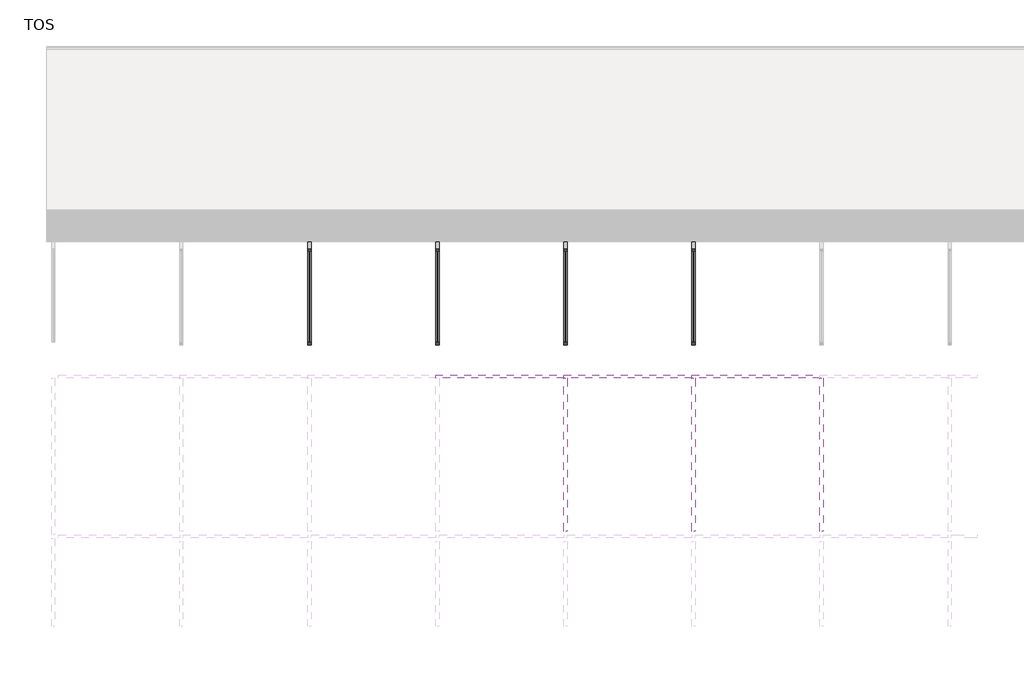
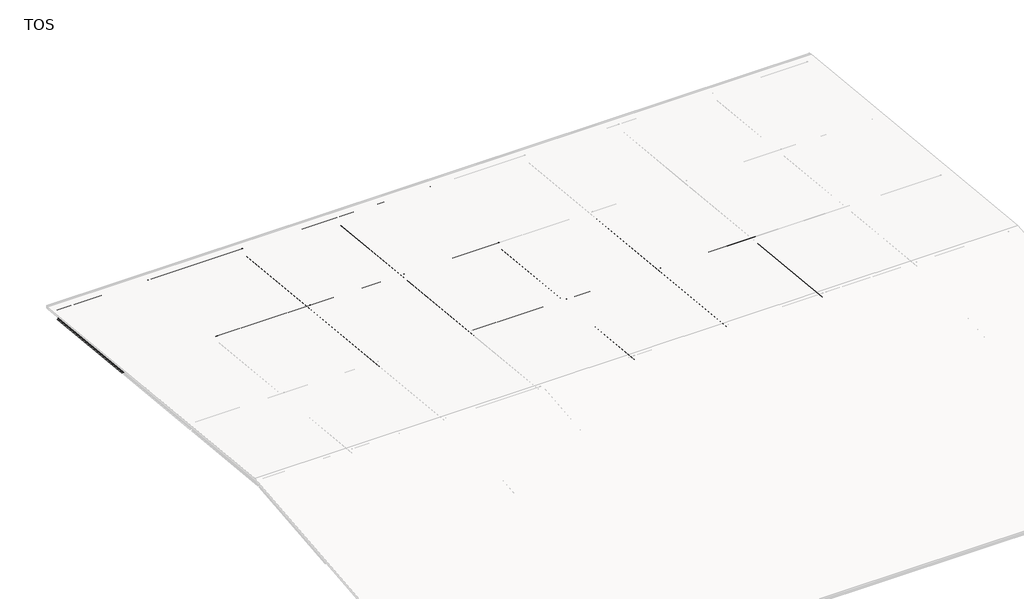
# One storey, part 4 of 5: 22 beams.
"""IFC4 building model written with IfcOpenShell, lengths in millimetres."""

from ifc_helpers import new_model, si_unit, point, frame, frame_2d, origin, place, context, project, spatial, polyline, circle_curve, trimmed, segment, composite_curve, outline, extrude, element, save

model = new_model("IFC4")

# Units and contexts
model_context = context("Model", 3, world=origin())
ifc_project = project(units=[si_unit("LENGTHUNIT", "METRE", prefix="MILLI")], contexts=[model_context])

# Site, building, storey
site = spatial("IfcSite", under=ifc_project)
building = spatial("IfcBuilding", under=site)
storey = spatial("IfcBuildingStorey", under=building, Name="TOS", Elevation=9299.9618634)

# Beams
placement = place(None, origin())
element("IfcBeam", 1, ObjectType="0912_Steel Framing_H-KSD3502 : H_SB_ASB_H-600x200x11x17", at=placement, inside=storey, context=model_context, shape_type="SweptSolid", body=[
    extrude(outline(composite_curve([segment(polyline([(40599.5208589, 10716.9618634), (40599.5208589, 10699.9618634), (40399.5208589, 10699.9618634), (40399.5208589, 10716.9618634), (40472.0208589, 10716.9618634)]), True, "CONTINUOUS"), segment(trimmed(circle_curve(frame_2d((40472.0208589, 10738.9618634)), 22.0), [point((40472.0208589, 10716.9618634))], [point((40494.0208589, 10738.9618634))], True, "CARTESIAN"), True, "CONTINUOUS"), segment(polyline([(40494.0208589, 10738.9618634), (40494.0208589, 11260.9618634)]), True, "CONTINUOUS"), segment(trimmed(circle_curve(frame_2d((40472.0208589, 11260.9618634)), 22.0), [point((40494.0208589, 11260.9618634))], [point((40472.0208589, 11282.9618634))], True, "CARTESIAN"), True, "CONTINUOUS"), segment(polyline([(40472.0208589, 11282.9618634), (40399.5208589, 11282.9618634), (40399.5208589, 11299.9618634), (40599.5208589, 11299.9618634), (40599.5208589, 11282.9618634), (40527.0208589, 11282.9618634)]), True, "CONTINUOUS"), segment(trimmed(circle_curve(frame_2d((40527.0208589, 11260.9618634)), 22.0), [point((40527.0208589, 11282.9618634))], [point((40505.0208589, 11260.9618634))], True, "CARTESIAN"), True, "CONTINUOUS"), segment(polyline([(40505.0208589, 11260.9618634), (40505.0208589, 10738.9618634)]), True, "CONTINUOUS"), segment(trimmed(circle_curve(frame_2d((40527.0208589, 10738.9618634)), 22.0), [point((40505.0208589, 10738.9618634))], [point((40527.0208589, 10716.9618634))], True, "CARTESIAN"), True, "CONTINUOUS"), segment(polyline([(40527.0208589, 10716.9618634), (40599.5208589, 10716.9618634)]), True, "CONTINUOUS")], self_intersect=False)), frame((23900.0, 0.0, 0.0), z_axis=(1.0, 0.0, 0.0), x_axis=(0.0, 1.0, 0.0)), (0.0, 0.0, 1.0), 7987.3),
])
element("IfcBeam", 2, ObjectType="0912_Steel Framing_H-KSD3502 : H_SB_ASB_H-600x200x11x17", at=placement, inside=storey, context=model_context, shape_type="SweptSolid", body=[
    extrude(outline(composite_curve([segment(polyline([(40599.5208589, 10716.9618634), (40599.5208589, 10699.9618634), (40399.5208589, 10699.9618634), (40399.5208589, 10716.9618634), (40472.0208589, 10716.9618634)]), True, "CONTINUOUS"), segment(trimmed(circle_curve(frame_2d((40472.0208589, 10738.9618634)), 22.0), [point((40472.0208589, 10716.9618634))], [point((40494.0208589, 10738.9618634))], True, "CARTESIAN"), True, "CONTINUOUS"), segment(polyline([(40494.0208589, 10738.9618634), (40494.0208589, 11260.9618634)]), True, "CONTINUOUS"), segment(trimmed(circle_curve(frame_2d((40472.0208589, 11260.9618634)), 22.0), [point((40494.0208589, 11260.9618634))], [point((40472.0208589, 11282.9618634))], True, "CARTESIAN"), True, "CONTINUOUS"), segment(polyline([(40472.0208589, 11282.9618634), (40399.5208589, 11282.9618634), (40399.5208589, 11299.9618634), (40599.5208589, 11299.9618634), (40599.5208589, 11282.9618634), (40527.0208589, 11282.9618634)]), True, "CONTINUOUS"), segment(trimmed(circle_curve(frame_2d((40527.0208589, 11260.9618634)), 22.0), [point((40527.0208589, 11282.9618634))], [point((40505.0208589, 11260.9618634))], True, "CARTESIAN"), True, "CONTINUOUS"), segment(polyline([(40505.0208589, 11260.9618634), (40505.0208589, 10738.9618634)]), True, "CONTINUOUS"), segment(trimmed(circle_curve(frame_2d((40527.0208589, 10738.9618634)), 22.0), [point((40505.0208589, 10738.9618634))], [point((40527.0208589, 10716.9618634))], True, "CARTESIAN"), True, "CONTINUOUS"), segment(polyline([(40527.0208589, 10716.9618634), (40599.5208589, 10716.9618634)]), True, "CONTINUOUS")], self_intersect=False)), frame((31900.0, 0.0, 0.0), z_axis=(1.0, 0.0, 0.0), x_axis=(0.0, 1.0, 0.0)), (0.0, 0.0, 1.0), 7987.3),
])
element("IfcBeam", 3, ObjectType="0912_Steel Framing_H-KSD3502 : H_SB_ASB_H-600x200x11x17", at=placement, inside=storey, context=model_context, shape_type="SweptSolid", body=[
    extrude(outline(composite_curve([segment(polyline([(40599.5208589, 10716.9618634), (40599.5208589, 10699.9618634), (40399.5208589, 10699.9618634), (40399.5208589, 10716.9618634), (40472.0208589, 10716.9618634)]), True, "CONTINUOUS"), segment(trimmed(circle_curve(frame_2d((40472.0208589, 10738.9618634)), 22.0), [point((40472.0208589, 10716.9618634))], [point((40494.0208589, 10738.9618634))], True, "CARTESIAN"), True, "CONTINUOUS"), segment(polyline([(40494.0208589, 10738.9618634), (40494.0208589, 11260.9618634)]), True, "CONTINUOUS"), segment(trimmed(circle_curve(frame_2d((40472.0208589, 11260.9618634)), 22.0), [point((40494.0208589, 11260.9618634))], [point((40472.0208589, 11282.9618634))], True, "CARTESIAN"), True, "CONTINUOUS"), segment(polyline([(40472.0208589, 11282.9618634), (40399.5208589, 11282.9618634), (40399.5208589, 11299.9618634), (40599.5208589, 11299.9618634), (40599.5208589, 11282.9618634), (40527.0208589, 11282.9618634)]), True, "CONTINUOUS"), segment(trimmed(circle_curve(frame_2d((40527.0208589, 11260.9618634)), 22.0), [point((40527.0208589, 11282.9618634))], [point((40505.0208589, 11260.9618634))], True, "CARTESIAN"), True, "CONTINUOUS"), segment(polyline([(40505.0208589, 11260.9618634), (40505.0208589, 10738.9618634)]), True, "CONTINUOUS"), segment(trimmed(circle_curve(frame_2d((40527.0208589, 10738.9618634)), 22.0), [point((40505.0208589, 10738.9618634))], [point((40527.0208589, 10716.9618634))], True, "CARTESIAN"), True, "CONTINUOUS"), segment(polyline([(40527.0208589, 10716.9618634), (40599.5208589, 10716.9618634)]), True, "CONTINUOUS")], self_intersect=False)), frame((39900.0, 0.0, 0.0), z_axis=(1.0, 0.0, 0.0), x_axis=(0.0, 1.0, 0.0)), (0.0, 0.0, 1.0), 7987.3),
])
element("IfcBeam", 4, ObjectType="0912_Steel Framing_H-KSD3502 : H_SB_ASB_H-600x200x11x17", at=placement, inside=storey, context=model_context, shape_type="SweptSolid", body=[
    extrude(outline(composite_curve([segment(polyline([(50599.5208589, 9716.9618634), (50599.5208589, 9699.9618634), (50399.5208589, 9699.9618634), (50399.5208589, 9716.9618634), (50472.0208589, 9716.9618634)]), True, "CONTINUOUS"), segment(trimmed(circle_curve(frame_2d((50472.0208589, 9738.9618634)), 22.0), [point((50472.0208589, 9716.9618634))], [point((50494.0208589, 9738.9618634))], True, "CARTESIAN"), True, "CONTINUOUS"), segment(polyline([(50494.0208589, 9738.9618634), (50494.0208589, 10260.9618634)]), True, "CONTINUOUS"), segment(trimmed(circle_curve(frame_2d((50472.0208589, 10260.9618634)), 22.0), [point((50494.0208589, 10260.9618634))], [point((50472.0208589, 10282.9618634))], True, "CARTESIAN"), True, "CONTINUOUS"), segment(polyline([(50472.0208589, 10282.9618634), (50399.5208589, 10282.9618634), (50399.5208589, 10299.9618634), (50599.5208589, 10299.9618634), (50599.5208589, 10282.9618634), (50527.0208589, 10282.9618634)]), True, "CONTINUOUS"), segment(trimmed(circle_curve(frame_2d((50527.0208589, 10260.9618634)), 22.0), [point((50527.0208589, 10282.9618634))], [point((50505.0208589, 10260.9618634))], True, "CARTESIAN"), True, "CONTINUOUS"), segment(polyline([(50505.0208589, 10260.9618634), (50505.0208589, 9738.9618634)]), True, "CONTINUOUS"), segment(trimmed(circle_curve(frame_2d((50527.0208589, 9738.9618634)), 22.0), [point((50505.0208589, 9738.9618634))], [point((50527.0208589, 9716.9618634))], True, "CARTESIAN"), True, "CONTINUOUS"), segment(polyline([(50527.0208589, 9716.9618634), (50599.5208589, 9716.9618634)]), True, "CONTINUOUS")], self_intersect=False)), frame((318.7, 0.0, 0.0), z_axis=(1.0, 0.0, 0.0), x_axis=(0.0, 1.0, 0.0)), (0.0, 0.0, 1.0), 7568.6),
])
element("IfcBeam", 5, ObjectType="0912_Steel Framing_H-KSD3502 : H_SB_ASB_H-600x200x11x17", at=placement, inside=storey, context=model_context, shape_type="SweptSolid", body=[
    extrude(outline(composite_curve([segment(polyline([(50599.5208589, 9716.9618634), (50599.5208589, 9699.9618634), (50399.5208589, 9699.9618634), (50399.5208589, 9716.9618634), (50472.0208589, 9716.9618634)]), True, "CONTINUOUS"), segment(trimmed(circle_curve(frame_2d((50472.0208589, 9738.9618634)), 22.0), [point((50472.0208589, 9716.9618634))], [point((50494.0208589, 9738.9618634))], True, "CARTESIAN"), True, "CONTINUOUS"), segment(polyline([(50494.0208589, 9738.9618634), (50494.0208589, 10260.9618634)]), True, "CONTINUOUS"), segment(trimmed(circle_curve(frame_2d((50472.0208589, 10260.9618634)), 22.0), [point((50494.0208589, 10260.9618634))], [point((50472.0208589, 10282.9618634))], True, "CARTESIAN"), True, "CONTINUOUS"), segment(polyline([(50472.0208589, 10282.9618634), (50399.5208589, 10282.9618634), (50399.5208589, 10299.9618634), (50599.5208589, 10299.9618634), (50599.5208589, 10282.9618634), (50527.0208589, 10282.9618634)]), True, "CONTINUOUS"), segment(trimmed(circle_curve(frame_2d((50527.0208589, 10260.9618634)), 22.0), [point((50527.0208589, 10282.9618634))], [point((50505.0208589, 10260.9618634))], True, "CARTESIAN"), True, "CONTINUOUS"), segment(polyline([(50505.0208589, 10260.9618634), (50505.0208589, 9738.9618634)]), True, "CONTINUOUS"), segment(trimmed(circle_curve(frame_2d((50527.0208589, 9738.9618634)), 22.0), [point((50505.0208589, 9738.9618634))], [point((50527.0208589, 9716.9618634))], True, "CARTESIAN"), True, "CONTINUOUS"), segment(polyline([(50527.0208589, 9716.9618634), (50599.5208589, 9716.9618634)]), True, "CONTINUOUS")], self_intersect=False)), frame((7900.0, 0.0, 0.0), z_axis=(1.0, 0.0, 0.0), x_axis=(0.0, 1.0, 0.0)), (0.0, 0.0, 1.0), 7987.3),
])
element("IfcBeam", 6, ObjectType="0912_Steel Framing_H-KSD3502 : H_SB_ASB_H-600x200x11x17", at=placement, inside=storey, context=model_context, shape_type="SweptSolid", body=[
    extrude(outline(composite_curve([segment(polyline([(50599.5208589, 9716.9618634), (50599.5208589, 9699.9618634), (50399.5208589, 9699.9618634), (50399.5208589, 9716.9618634), (50472.0208589, 9716.9618634)]), True, "CONTINUOUS"), segment(trimmed(circle_curve(frame_2d((50472.0208589, 9738.9618634)), 22.0), [point((50472.0208589, 9716.9618634))], [point((50494.0208589, 9738.9618634))], True, "CARTESIAN"), True, "CONTINUOUS"), segment(polyline([(50494.0208589, 9738.9618634), (50494.0208589, 10260.9618634)]), True, "CONTINUOUS"), segment(trimmed(circle_curve(frame_2d((50472.0208589, 10260.9618634)), 22.0), [point((50494.0208589, 10260.9618634))], [point((50472.0208589, 10282.9618634))], True, "CARTESIAN"), True, "CONTINUOUS"), segment(polyline([(50472.0208589, 10282.9618634), (50399.5208589, 10282.9618634), (50399.5208589, 10299.9618634), (50599.5208589, 10299.9618634), (50599.5208589, 10282.9618634), (50527.0208589, 10282.9618634)]), True, "CONTINUOUS"), segment(trimmed(circle_curve(frame_2d((50527.0208589, 10260.9618634)), 22.0), [point((50527.0208589, 10282.9618634))], [point((50505.0208589, 10260.9618634))], True, "CARTESIAN"), True, "CONTINUOUS"), segment(polyline([(50505.0208589, 10260.9618634), (50505.0208589, 9738.9618634)]), True, "CONTINUOUS"), segment(trimmed(circle_curve(frame_2d((50527.0208589, 9738.9618634)), 22.0), [point((50505.0208589, 9738.9618634))], [point((50527.0208589, 9716.9618634))], True, "CARTESIAN"), True, "CONTINUOUS"), segment(polyline([(50527.0208589, 9716.9618634), (50599.5208589, 9716.9618634)]), True, "CONTINUOUS")], self_intersect=False)), frame((15900.0, 0.0, 0.0), z_axis=(1.0, 0.0, 0.0), x_axis=(0.0, 1.0, 0.0)), (0.0, 0.0, 1.0), 7987.3),
])
element("IfcBeam", 7, ObjectType="0912_Steel Framing_H-KSD3502 : H_SB_ASB_H-600x200x11x17", at=placement, inside=storey, context=model_context, shape_type="SweptSolid", body=[
    extrude(outline(composite_curve([segment(polyline([(50599.5208589, 9716.9618634), (50599.5208589, 9699.9618634), (50399.5208589, 9699.9618634), (50399.5208589, 9716.9618634), (50472.0208589, 9716.9618634)]), True, "CONTINUOUS"), segment(trimmed(circle_curve(frame_2d((50472.0208589, 9738.9618634)), 22.0), [point((50472.0208589, 9716.9618634))], [point((50494.0208589, 9738.9618634))], True, "CARTESIAN"), True, "CONTINUOUS"), segment(polyline([(50494.0208589, 9738.9618634), (50494.0208589, 10260.9618634)]), True, "CONTINUOUS"), segment(trimmed(circle_curve(frame_2d((50472.0208589, 10260.9618634)), 22.0), [point((50494.0208589, 10260.9618634))], [point((50472.0208589, 10282.9618634))], True, "CARTESIAN"), True, "CONTINUOUS"), segment(polyline([(50472.0208589, 10282.9618634), (50399.5208589, 10282.9618634), (50399.5208589, 10299.9618634), (50599.5208589, 10299.9618634), (50599.5208589, 10282.9618634), (50527.0208589, 10282.9618634)]), True, "CONTINUOUS"), segment(trimmed(circle_curve(frame_2d((50527.0208589, 10260.9618634)), 22.0), [point((50527.0208589, 10282.9618634))], [point((50505.0208589, 10260.9618634))], True, "CARTESIAN"), True, "CONTINUOUS"), segment(polyline([(50505.0208589, 10260.9618634), (50505.0208589, 9738.9618634)]), True, "CONTINUOUS"), segment(trimmed(circle_curve(frame_2d((50527.0208589, 9738.9618634)), 22.0), [point((50505.0208589, 9738.9618634))], [point((50527.0208589, 9716.9618634))], True, "CARTESIAN"), True, "CONTINUOUS"), segment(polyline([(50527.0208589, 9716.9618634), (50599.5208589, 9716.9618634)]), True, "CONTINUOUS")], self_intersect=False)), frame((23900.0, 0.0, 0.0), z_axis=(1.0, 0.0, 0.0), x_axis=(0.0, 1.0, 0.0)), (0.0, 0.0, 1.0), 7987.3),
])
element("IfcBeam", 8, ObjectType="0912_Steel Framing_H-KSD3502 : H_SB_ASB_H-600x200x11x17", at=placement, inside=storey, context=model_context, shape_type="SweptSolid", body=[
    extrude(outline(composite_curve([segment(polyline([(60599.5208589, 8716.9618634), (60599.5208589, 8699.9618634), (60399.5208589, 8699.9618634), (60399.5208589, 8716.9618634), (60472.0208589, 8716.9618634)]), True, "CONTINUOUS"), segment(trimmed(circle_curve(frame_2d((60472.0208589, 8738.9618634)), 22.0), [point((60472.0208589, 8716.9618634))], [point((60494.0208589, 8738.9618634))], True, "CARTESIAN"), True, "CONTINUOUS"), segment(polyline([(60494.0208589, 8738.9618634), (60494.0208589, 9260.9618634)]), True, "CONTINUOUS"), segment(trimmed(circle_curve(frame_2d((60472.0208589, 9260.9618634)), 22.0), [point((60494.0208589, 9260.9618634))], [point((60472.0208589, 9282.9618634))], True, "CARTESIAN"), True, "CONTINUOUS"), segment(polyline([(60472.0208589, 9282.9618634), (60399.5208589, 9282.9618634), (60399.5208589, 9299.9618634), (60599.5208589, 9299.9618634), (60599.5208589, 9282.9618634), (60527.0208589, 9282.9618634)]), True, "CONTINUOUS"), segment(trimmed(circle_curve(frame_2d((60527.0208589, 9260.9618634)), 22.0), [point((60527.0208589, 9282.9618634))], [point((60505.0208589, 9260.9618634))], True, "CARTESIAN"), True, "CONTINUOUS"), segment(polyline([(60505.0208589, 9260.9618634), (60505.0208589, 8738.9618634)]), True, "CONTINUOUS"), segment(trimmed(circle_curve(frame_2d((60527.0208589, 8738.9618634)), 22.0), [point((60505.0208589, 8738.9618634))], [point((60527.0208589, 8716.9618634))], True, "CARTESIAN"), True, "CONTINUOUS"), segment(polyline([(60527.0208589, 8716.9618634), (60599.5208589, 8716.9618634)]), True, "CONTINUOUS")], self_intersect=False)), frame((113.7, 0.0, 0.0), z_axis=(1.0, 0.0, 0.0), x_axis=(0.0, 1.0, 0.0)), (0.0, 0.0, 1.0), 7772.6),
])
element("IfcBeam", 9, ObjectType="0912_Steel Framing_H-KSD3502 : H_SB_ASB_H-600x200x11x17", at=placement, inside=storey, context=model_context, shape_type="SweptSolid", body=[
    extrude(outline(composite_curve([segment(polyline([(60599.5208589, 8716.9618634), (60599.5208589, 8699.9618634), (60399.5208589, 8699.9618634), (60399.5208589, 8716.9618634), (60472.0208589, 8716.9618634)]), True, "CONTINUOUS"), segment(trimmed(circle_curve(frame_2d((60472.0208589, 8738.9618634)), 22.0), [point((60472.0208589, 8716.9618634))], [point((60494.0208589, 8738.9618634))], True, "CARTESIAN"), True, "CONTINUOUS"), segment(polyline([(60494.0208589, 8738.9618634), (60494.0208589, 9260.9618634)]), True, "CONTINUOUS"), segment(trimmed(circle_curve(frame_2d((60472.0208589, 9260.9618634)), 22.0), [point((60494.0208589, 9260.9618634))], [point((60472.0208589, 9282.9618634))], True, "CARTESIAN"), True, "CONTINUOUS"), segment(polyline([(60472.0208589, 9282.9618634), (60399.5208589, 9282.9618634), (60399.5208589, 9299.9618634), (60599.5208589, 9299.9618634), (60599.5208589, 9282.9618634), (60527.0208589, 9282.9618634)]), True, "CONTINUOUS"), segment(trimmed(circle_curve(frame_2d((60527.0208589, 9260.9618634)), 22.0), [point((60527.0208589, 9282.9618634))], [point((60505.0208589, 9260.9618634))], True, "CARTESIAN"), True, "CONTINUOUS"), segment(polyline([(60505.0208589, 9260.9618634), (60505.0208589, 8738.9618634)]), True, "CONTINUOUS"), segment(trimmed(circle_curve(frame_2d((60527.0208589, 8738.9618634)), 22.0), [point((60505.0208589, 8738.9618634))], [point((60527.0208589, 8716.9618634))], True, "CARTESIAN"), True, "CONTINUOUS"), segment(polyline([(60527.0208589, 8716.9618634), (60599.5208589, 8716.9618634)]), True, "CONTINUOUS")], self_intersect=False)), frame((8113.7, 0.0, 0.0), z_axis=(1.0, 0.0, 0.0), x_axis=(0.0, 1.0, 0.0)), (0.0, 0.0, 1.0), 7772.6),
])
element("IfcBeam", 10, ObjectType="0912_Steel Framing_H-KSD3502 : H_SB_ASB_H-600x200x11x17", at=placement, inside=storey, context=model_context, shape_type="SweptSolid", body=[
    extrude(outline(composite_curve([segment(polyline([(60599.5208589, 8716.9618634), (60599.5208589, 8699.9618634), (60399.5208589, 8699.9618634), (60399.5208589, 8716.9618634), (60472.0208589, 8716.9618634)]), True, "CONTINUOUS"), segment(trimmed(circle_curve(frame_2d((60472.0208589, 8738.9618634)), 22.0), [point((60472.0208589, 8716.9618634))], [point((60494.0208589, 8738.9618634))], True, "CARTESIAN"), True, "CONTINUOUS"), segment(polyline([(60494.0208589, 8738.9618634), (60494.0208589, 9260.9618634)]), True, "CONTINUOUS"), segment(trimmed(circle_curve(frame_2d((60472.0208589, 9260.9618634)), 22.0), [point((60494.0208589, 9260.9618634))], [point((60472.0208589, 9282.9618634))], True, "CARTESIAN"), True, "CONTINUOUS"), segment(polyline([(60472.0208589, 9282.9618634), (60399.5208589, 9282.9618634), (60399.5208589, 9299.9618634), (60599.5208589, 9299.9618634), (60599.5208589, 9282.9618634), (60527.0208589, 9282.9618634)]), True, "CONTINUOUS"), segment(trimmed(circle_curve(frame_2d((60527.0208589, 9260.9618634)), 22.0), [point((60527.0208589, 9282.9618634))], [point((60505.0208589, 9260.9618634))], True, "CARTESIAN"), True, "CONTINUOUS"), segment(polyline([(60505.0208589, 9260.9618634), (60505.0208589, 8738.9618634)]), True, "CONTINUOUS"), segment(trimmed(circle_curve(frame_2d((60527.0208589, 8738.9618634)), 22.0), [point((60505.0208589, 8738.9618634))], [point((60527.0208589, 8716.9618634))], True, "CARTESIAN"), True, "CONTINUOUS"), segment(polyline([(60527.0208589, 8716.9618634), (60599.5208589, 8716.9618634)]), True, "CONTINUOUS")], self_intersect=False)), frame((16113.7, 0.0, 0.0), z_axis=(1.0, 0.0, 0.0), x_axis=(0.0, 1.0, 0.0)), (0.0, 0.0, 1.0), 7772.6),
])
element("IfcBeam", 11, ObjectType="0912_Steel Framing_H-KSD3502 : H_SB_ASB_H-600x200x11x17", at=placement, inside=storey, context=model_context, shape_type="SweptSolid", body=[
    extrude(outline(composite_curve([segment(polyline([(60599.5208589, 8716.9618634), (60599.5208589, 8699.9618634), (60399.5208589, 8699.9618634), (60399.5208589, 8716.9618634), (60472.0208589, 8716.9618634)]), True, "CONTINUOUS"), segment(trimmed(circle_curve(frame_2d((60472.0208589, 8738.9618634)), 22.0), [point((60472.0208589, 8716.9618634))], [point((60494.0208589, 8738.9618634))], True, "CARTESIAN"), True, "CONTINUOUS"), segment(polyline([(60494.0208589, 8738.9618634), (60494.0208589, 9260.9618634)]), True, "CONTINUOUS"), segment(trimmed(circle_curve(frame_2d((60472.0208589, 9260.9618634)), 22.0), [point((60494.0208589, 9260.9618634))], [point((60472.0208589, 9282.9618634))], True, "CARTESIAN"), True, "CONTINUOUS"), segment(polyline([(60472.0208589, 9282.9618634), (60399.5208589, 9282.9618634), (60399.5208589, 9299.9618634), (60599.5208589, 9299.9618634), (60599.5208589, 9282.9618634), (60527.0208589, 9282.9618634)]), True, "CONTINUOUS"), segment(trimmed(circle_curve(frame_2d((60527.0208589, 9260.9618634)), 22.0), [point((60527.0208589, 9282.9618634))], [point((60505.0208589, 9260.9618634))], True, "CARTESIAN"), True, "CONTINUOUS"), segment(polyline([(60505.0208589, 9260.9618634), (60505.0208589, 8738.9618634)]), True, "CONTINUOUS"), segment(trimmed(circle_curve(frame_2d((60527.0208589, 8738.9618634)), 22.0), [point((60505.0208589, 8738.9618634))], [point((60527.0208589, 8716.9618634))], True, "CARTESIAN"), True, "CONTINUOUS"), segment(polyline([(60527.0208589, 8716.9618634), (60599.5208589, 8716.9618634)]), True, "CONTINUOUS")], self_intersect=False)), frame((24113.7, 0.0, 0.0), z_axis=(1.0, 0.0, 0.0), x_axis=(0.0, 1.0, 0.0)), (0.0, 0.0, 1.0), 7772.6),
])
element("IfcBeam", 12, ObjectType="0912_Steel Framing_H-KSD3502 : H_SB_ASB_H-600x200x11x17", at=placement, inside=storey, context=model_context, shape_type="SweptSolid", body=[
    extrude(outline(composite_curve([segment(polyline([(-283.0, 100.0), (-283.0, 27.5)]), True, "CONTINUOUS"), segment(trimmed(circle_curve(frame_2d((-260.9999999, 27.5)), 22.0), [point((-283.0, 27.5))], [point((-260.9999999, 5.5))], True, "CARTESIAN"), True, "CONTINUOUS"), segment(polyline([(-260.9999999, 5.5), (261.0000001, 5.5)]), True, "CONTINUOUS"), segment(trimmed(circle_curve(frame_2d((261.0000001, 27.5)), 22.0), [point((261.0000001, 5.5))], [point((283.0000001, 27.5))], True, "CARTESIAN"), True, "CONTINUOUS"), segment(polyline([(283.0000001, 27.5), (283.0000001, 100.0), (300.0, 100.0), (300.0, -100.0), (283.0000001, -100.0), (283.0000001, -27.5)]), True, "CONTINUOUS"), segment(trimmed(circle_curve(frame_2d((261.0000001, -27.5)), 22.0), [point((283.0000001, -27.5))], [point((261.0000001, -5.5))], True, "CARTESIAN"), True, "CONTINUOUS"), segment(polyline([(261.0000001, -5.5), (-260.9999999, -5.5)]), True, "CONTINUOUS"), segment(trimmed(circle_curve(frame_2d((-260.9999999, -27.5)), 22.0), [point((-260.9999999, -5.5))], [point((-283.0, -27.5))], True, "CARTESIAN"), True, "CONTINUOUS"), segment(polyline([(-283.0, -27.5), (-283.0, -100.0), (-299.9999999, -100.0), (-299.9999999, 100.0), (-283.0, 100.0)]), True, "CONTINUOUS")], self_intersect=False)), frame((0.0, 60154.0624738, 9033.0114332), z_axis=(0.0, -0.9950371902099892, 0.09950371902099907), x_axis=(0.0, 0.09950371902099907, 0.9950371902099892)), (0.0, 0.0, 1.0), 9558.4904971),
])
element("IfcBeam", 13, ObjectType="0912_Steel Framing_H-KSD3502 : H_SB_ASB_H-600x200x11x17", at=placement, inside=storey, context=model_context, shape_type="SweptSolid", body=[
    extrude(outline(composite_curve([segment(polyline([(-283.0, 100.0), (-283.0, 27.5)]), True, "CONTINUOUS"), segment(trimmed(circle_curve(frame_2d((-260.9999999, 27.5)), 22.0), [point((-283.0, 27.5))], [point((-260.9999999, 5.5))], True, "CARTESIAN"), True, "CONTINUOUS"), segment(polyline([(-260.9999999, 5.5), (261.0000001, 5.5)]), True, "CONTINUOUS"), segment(trimmed(circle_curve(frame_2d((261.0000001, 27.5)), 22.0), [point((261.0000001, 5.5))], [point((283.0000001, 27.5))], True, "CARTESIAN"), True, "CONTINUOUS"), segment(polyline([(283.0000001, 27.5), (283.0000001, 100.0), (300.0, 100.0), (300.0, -100.0), (283.0000001, -100.0), (283.0000001, -27.5)]), True, "CONTINUOUS"), segment(trimmed(circle_curve(frame_2d((261.0000001, -27.5)), 22.0), [point((283.0000001, -27.5))], [point((261.0000001, -5.5))], True, "CARTESIAN"), True, "CONTINUOUS"), segment(polyline([(261.0000001, -5.5), (-260.9999999, -5.5)]), True, "CONTINUOUS"), segment(trimmed(circle_curve(frame_2d((-260.9999999, -27.5)), 22.0), [point((-260.9999999, -5.5))], [point((-283.0, -27.5))], True, "CARTESIAN"), True, "CONTINUOUS"), segment(polyline([(-283.0, -27.5), (-283.0, -100.0), (-299.9999999, -100.0), (-299.9999999, 100.0), (-283.0, 100.0)]), True, "CONTINUOUS")], self_intersect=False)), frame((8000.0, 60154.0624738, 9033.0114332), z_axis=(0.0, -0.9950371902099892, 0.09950371902099907), x_axis=(0.0, 0.09950371902099907, 0.9950371902099892)), (0.0, 0.0, 1.0), 9560.7882905),
])
element("IfcBeam", 14, ObjectType="0912_Steel Framing_H-KSD3502 : H_SB_ASB_H-600x200x11x17", at=placement, inside=storey, context=model_context, shape_type="SweptSolid", body=[
    extrude(outline(composite_curve([segment(polyline([(-283.0, 100.0), (-283.0, 27.5)]), True, "CONTINUOUS"), segment(trimmed(circle_curve(frame_2d((-261.0, 27.5)), 22.0), [point((-283.0, 27.5))], [point((-261.0, 5.5))], True, "CARTESIAN"), True, "CONTINUOUS"), segment(polyline([(-261.0, 5.5), (261.0, 5.5)]), True, "CONTINUOUS"), segment(trimmed(circle_curve(frame_2d((261.0, 27.5)), 22.0), [point((261.0, 5.5))], [point((283.0000001, 27.5))], True, "CARTESIAN"), True, "CONTINUOUS"), segment(polyline([(283.0000001, 27.5), (283.0000001, 100.0), (300.0, 100.0), (300.0, -100.0), (283.0000001, -100.0), (283.0000001, -27.5)]), True, "CONTINUOUS"), segment(trimmed(circle_curve(frame_2d((261.0, -27.5)), 22.0), [point((283.0000001, -27.5))], [point((261.0, -5.5))], True, "CARTESIAN"), True, "CONTINUOUS"), segment(polyline([(261.0, -5.5), (-261.0, -5.5)]), True, "CONTINUOUS"), segment(trimmed(circle_curve(frame_2d((-261.0, -27.5)), 22.0), [point((-261.0, -5.5))], [point((-283.0, -27.5))], True, "CARTESIAN"), True, "CONTINUOUS"), segment(polyline([(-283.0, -27.5), (-283.0, -100.0), (-299.9999999, -100.0), (-299.9999999, 100.0), (-283.0, 100.0)]), True, "CONTINUOUS")], self_intersect=False)), frame((16000.0, 50358.0228699, 10012.6153936), z_axis=(0.0, -0.9950371902099892, 0.09950371902099896), x_axis=(0.0, 0.09950371902099896, 0.9950371902099892)), (0.0, 0.0, 1.0), 9765.7659517),
])
element("IfcBeam", 15, ObjectType="0912_Steel Framing_H-KSD3502 : H_SB_ASB_H-600x200x11x17", at=placement, inside=storey, context=model_context, shape_type="SweptSolid", body=[
    extrude(outline(composite_curve([segment(polyline([(-283.0, 100.0), (-283.0, 27.5)]), True, "CONTINUOUS"), segment(trimmed(circle_curve(frame_2d((-260.9999999, 27.5)), 22.0), [point((-283.0, 27.5))], [point((-260.9999999, 5.5))], True, "CARTESIAN"), True, "CONTINUOUS"), segment(polyline([(-260.9999999, 5.5), (261.0000001, 5.5)]), True, "CONTINUOUS"), segment(trimmed(circle_curve(frame_2d((261.0000001, 27.5)), 22.0), [point((261.0000001, 5.5))], [point((283.0000001, 27.5))], True, "CARTESIAN"), True, "CONTINUOUS"), segment(polyline([(283.0000001, 27.5), (283.0000001, 100.0), (300.0, 100.0), (300.0, -100.0), (283.0000001, -100.0), (283.0000001, -27.5)]), True, "CONTINUOUS"), segment(trimmed(circle_curve(frame_2d((261.0000001, -27.5)), 22.0), [point((283.0000001, -27.5))], [point((261.0000001, -5.5))], True, "CARTESIAN"), True, "CONTINUOUS"), segment(polyline([(261.0000001, -5.5), (-260.9999999, -5.5)]), True, "CONTINUOUS"), segment(trimmed(circle_curve(frame_2d((-260.9999999, -27.5)), 22.0), [point((-260.9999999, -5.5))], [point((-283.0, -27.5))], True, "CARTESIAN"), True, "CONTINUOUS"), segment(polyline([(-283.0, -27.5), (-283.0, -100.0), (-299.9999999, -100.0), (-299.9999999, 100.0), (-283.0, 100.0)]), True, "CONTINUOUS")], self_intersect=False)), frame((16000.0, 60154.0624738, 9033.0114332), z_axis=(0.0, -0.9950371902099892, 0.09950371902099907), x_axis=(0.0, 0.09950371902099907, 0.9950371902099892)), (0.0, 0.0, 1.0), 9560.7882905),
])
element("IfcBeam", 16, ObjectType="0912_Steel Framing_H-KSD3502 : H_SB_ASB_H-600x200x11x17", at=placement, inside=storey, context=model_context, shape_type="SweptSolid", body=[
    extrude(outline(composite_curve([segment(polyline([(-283.0, 100.0), (-283.0, 27.5)]), True, "CONTINUOUS"), segment(trimmed(circle_curve(frame_2d((-261.0, 27.5)), 22.0), [point((-283.0, 27.5))], [point((-261.0, 5.5))], True, "CARTESIAN"), True, "CONTINUOUS"), segment(polyline([(-261.0, 5.5), (261.0, 5.5)]), True, "CONTINUOUS"), segment(trimmed(circle_curve(frame_2d((261.0, 27.5)), 22.0), [point((261.0, 5.5))], [point((283.0000001, 27.5))], True, "CARTESIAN"), True, "CONTINUOUS"), segment(polyline([(283.0000001, 27.5), (283.0000001, 100.0), (300.0, 100.0), (300.0, -100.0), (283.0000001, -100.0), (283.0000001, -27.5)]), True, "CONTINUOUS"), segment(trimmed(circle_curve(frame_2d((261.0, -27.5)), 22.0), [point((283.0000001, -27.5))], [point((261.0, -5.5))], True, "CARTESIAN"), True, "CONTINUOUS"), segment(polyline([(261.0, -5.5), (-261.0, -5.5)]), True, "CONTINUOUS"), segment(trimmed(circle_curve(frame_2d((-261.0, -27.5)), 22.0), [point((-261.0, -5.5))], [point((-283.0, -27.5))], True, "CARTESIAN"), True, "CONTINUOUS"), segment(polyline([(-283.0, -27.5), (-283.0, -100.0), (-299.9999999, -100.0), (-299.9999999, 100.0), (-283.0, 100.0)]), True, "CONTINUOUS")], self_intersect=False)), frame((24000.0, 50358.0228699, 10012.6153936), z_axis=(0.0, -0.9950371902099892, 0.09950371902099896), x_axis=(0.0, 0.09950371902099896, 0.9950371902099892)), (0.0, 0.0, 1.0), 9765.7659517),
])
element("IfcBeam", 17, ObjectType="0912_Steel Framing_H-KSD3502 : H_SB_ASB_H-600x200x11x17", at=placement, inside=storey, context=model_context, shape_type="SweptSolid", body=[
    extrude(outline(composite_curve([segment(polyline([(-283.0, 100.0), (-283.0, 27.5)]), True, "CONTINUOUS"), segment(trimmed(circle_curve(frame_2d((-260.9999999, 27.5)), 22.0), [point((-283.0, 27.5))], [point((-260.9999999, 5.5))], True, "CARTESIAN"), True, "CONTINUOUS"), segment(polyline([(-260.9999999, 5.5), (261.0000001, 5.5)]), True, "CONTINUOUS"), segment(trimmed(circle_curve(frame_2d((261.0000001, 27.5)), 22.0), [point((261.0000001, 5.5))], [point((283.0000001, 27.5))], True, "CARTESIAN"), True, "CONTINUOUS"), segment(polyline([(283.0000001, 27.5), (283.0000001, 100.0), (300.0, 100.0), (300.0, -100.0), (283.0000001, -100.0), (283.0000001, -27.5)]), True, "CONTINUOUS"), segment(trimmed(circle_curve(frame_2d((261.0000001, -27.5)), 22.0), [point((283.0000001, -27.5))], [point((261.0000001, -5.5))], True, "CARTESIAN"), True, "CONTINUOUS"), segment(polyline([(261.0000001, -5.5), (-260.9999999, -5.5)]), True, "CONTINUOUS"), segment(trimmed(circle_curve(frame_2d((-260.9999999, -27.5)), 22.0), [point((-260.9999999, -5.5))], [point((-283.0, -27.5))], True, "CARTESIAN"), True, "CONTINUOUS"), segment(polyline([(-283.0, -27.5), (-283.0, -100.0), (-299.9999999, -100.0), (-299.9999999, 100.0), (-283.0, 100.0)]), True, "CONTINUOUS")], self_intersect=False)), frame((24000.0, 60154.0624738, 9033.0114332), z_axis=(0.0, -0.9950371902099892, 0.09950371902099907), x_axis=(0.0, 0.09950371902099907, 0.9950371902099892)), (0.0, 0.0, 1.0), 9560.7882905),
])
element("IfcBeam", 18, ObjectType="0912_Steel Framing_H-KSD3502 : H_SB_ASB_H-600x200x11x17", at=placement, inside=storey, context=model_context, shape_type="SweptSolid", body=[
    extrude(outline(composite_curve([segment(polyline([(-283.0, 100.0), (-283.0, 27.5)]), True, "CONTINUOUS"), segment(trimmed(circle_curve(frame_2d((-261.0, 27.5)), 22.0), [point((-283.0, 27.5))], [point((-261.0, 5.5))], True, "CARTESIAN"), True, "CONTINUOUS"), segment(polyline([(-261.0, 5.5), (261.0, 5.5)]), True, "CONTINUOUS"), segment(trimmed(circle_curve(frame_2d((261.0, 27.5)), 22.0), [point((261.0, 5.5))], [point((283.0000001, 27.5))], True, "CARTESIAN"), True, "CONTINUOUS"), segment(polyline([(283.0000001, 27.5), (283.0000001, 100.0), (300.0, 100.0), (300.0, -100.0), (283.0000001, -100.0), (283.0000001, -27.5)]), True, "CONTINUOUS"), segment(trimmed(circle_curve(frame_2d((261.0, -27.5)), 22.0), [point((283.0000001, -27.5))], [point((261.0, -5.5))], True, "CARTESIAN"), True, "CONTINUOUS"), segment(polyline([(261.0, -5.5), (-261.0, -5.5)]), True, "CONTINUOUS"), segment(trimmed(circle_curve(frame_2d((-261.0, -27.5)), 22.0), [point((-261.0, -5.5))], [point((-283.0, -27.5))], True, "CARTESIAN"), True, "CONTINUOUS"), segment(polyline([(-283.0, -27.5), (-283.0, -100.0), (-299.9999999, -100.0), (-299.9999999, 100.0), (-283.0, 100.0)]), True, "CONTINUOUS")], self_intersect=False)), frame((32000.0, 40358.0228699, 11012.6153936), z_axis=(0.0, -0.9950371902099892, 0.09950371902099896), x_axis=(0.0, 0.09950371902099896, 0.9950371902099892)), (0.0, 0.0, 1.0), 9557.4457081),
])
element("IfcBeam", 19, ObjectType="0912_Steel Framing_H-KSD3502 : H_SB_ASB_H-600x200x11x17", at=placement, inside=storey, context=model_context, shape_type="SweptSolid", body=[
    extrude(outline(composite_curve([segment(polyline([(-283.0, 100.0), (-283.0, 27.5)]), True, "CONTINUOUS"), segment(trimmed(circle_curve(frame_2d((-261.0, 27.5)), 22.0), [point((-283.0, 27.5))], [point((-261.0, 5.5))], True, "CARTESIAN"), True, "CONTINUOUS"), segment(polyline([(-261.0, 5.5), (261.0, 5.5)]), True, "CONTINUOUS"), segment(trimmed(circle_curve(frame_2d((261.0, 27.5)), 22.0), [point((261.0, 5.5))], [point((283.0000001, 27.5))], True, "CARTESIAN"), True, "CONTINUOUS"), segment(polyline([(283.0000001, 27.5), (283.0000001, 100.0), (300.0, 100.0), (300.0, -100.0), (283.0000001, -100.0), (283.0000001, -27.5)]), True, "CONTINUOUS"), segment(trimmed(circle_curve(frame_2d((261.0, -27.5)), 22.0), [point((283.0000001, -27.5))], [point((261.0, -5.5))], True, "CARTESIAN"), True, "CONTINUOUS"), segment(polyline([(261.0, -5.5), (-261.0, -5.5)]), True, "CONTINUOUS"), segment(trimmed(circle_curve(frame_2d((-261.0, -27.5)), 22.0), [point((-261.0, -5.5))], [point((-283.0, -27.5))], True, "CARTESIAN"), True, "CONTINUOUS"), segment(polyline([(-283.0, -27.5), (-283.0, -100.0), (-299.9999999, -100.0), (-299.9999999, 100.0), (-283.0, 100.0)]), True, "CONTINUOUS")], self_intersect=False)), frame((32000.0, 50358.0228699, 10012.6153936), z_axis=(0.0, -0.9950371902099892, 0.09950371902099896), x_axis=(0.0, 0.09950371902099896, 0.9950371902099892)), (0.0, 0.0, 1.0), 9765.7659517),
])
element("IfcBeam", 20, ObjectType="0912_Steel Framing_H-KSD3502 : H_SB_ASB_H-600x200x11x17", at=placement, inside=storey, context=model_context, shape_type="SweptSolid", body=[
    extrude(outline(composite_curve([segment(polyline([(-283.0, 100.0), (-283.0, 27.5)]), True, "CONTINUOUS"), segment(trimmed(circle_curve(frame_2d((-261.0, 27.5)), 22.0), [point((-283.0, 27.5))], [point((-261.0, 5.5))], True, "CARTESIAN"), True, "CONTINUOUS"), segment(polyline([(-261.0, 5.5), (261.0, 5.5)]), True, "CONTINUOUS"), segment(trimmed(circle_curve(frame_2d((261.0, 27.5)), 22.0), [point((261.0, 5.5))], [point((283.0000001, 27.5))], True, "CARTESIAN"), True, "CONTINUOUS"), segment(polyline([(283.0000001, 27.5), (283.0000001, 100.0), (300.0, 100.0), (300.0, -100.0), (283.0000001, -100.0), (283.0000001, -27.5)]), True, "CONTINUOUS"), segment(trimmed(circle_curve(frame_2d((261.0, -27.5)), 22.0), [point((283.0000001, -27.5))], [point((261.0, -5.5))], True, "CARTESIAN"), True, "CONTINUOUS"), segment(polyline([(261.0, -5.5), (-261.0, -5.5)]), True, "CONTINUOUS"), segment(trimmed(circle_curve(frame_2d((-261.0, -27.5)), 22.0), [point((-261.0, -5.5))], [point((-283.0, -27.5))], True, "CARTESIAN"), True, "CONTINUOUS"), segment(polyline([(-283.0, -27.5), (-283.0, -100.0), (-299.9999999, -100.0), (-299.9999999, 100.0), (-283.0, 100.0)]), True, "CONTINUOUS")], self_intersect=False)), frame((40000.0, 40358.0228699, 11012.6153936), z_axis=(0.0, -0.9950371902099892, 0.09950371902099892), x_axis=(0.0, 0.09950371902099892, 0.9950371902099892)), (0.0, 0.0, 1.0), 9557.4457081),
])
element("IfcBeam", 21, ObjectType="0912_Steel Framing_H-KSD3502 : H_SB_ASB_H-600x200x11x17", at=placement, inside=storey, context=model_context, shape_type="SweptSolid", body=[
    extrude(outline(composite_curve([segment(polyline([(-283.0, 100.0), (-283.0, 27.5)]), True, "CONTINUOUS"), segment(trimmed(circle_curve(frame_2d((-261.0, 27.5)), 22.0), [point((-283.0, 27.5))], [point((-261.0, 5.5))], True, "CARTESIAN"), True, "CONTINUOUS"), segment(polyline([(-261.0, 5.5), (261.0, 5.5)]), True, "CONTINUOUS"), segment(trimmed(circle_curve(frame_2d((261.0, 27.5)), 22.0), [point((261.0, 5.5))], [point((283.0000001, 27.5))], True, "CARTESIAN"), True, "CONTINUOUS"), segment(polyline([(283.0000001, 27.5), (283.0000001, 100.0), (300.0, 100.0), (300.0, -100.0), (283.0000001, -100.0), (283.0000001, -27.5)]), True, "CONTINUOUS"), segment(trimmed(circle_curve(frame_2d((261.0, -27.5)), 22.0), [point((283.0000001, -27.5))], [point((261.0, -5.5))], True, "CARTESIAN"), True, "CONTINUOUS"), segment(polyline([(261.0, -5.5), (-261.0, -5.5)]), True, "CONTINUOUS"), segment(trimmed(circle_curve(frame_2d((-261.0, -27.5)), 22.0), [point((-261.0, -5.5))], [point((-283.0, -27.5))], True, "CARTESIAN"), True, "CONTINUOUS"), segment(polyline([(-283.0, -27.5), (-283.0, -100.0), (-299.9999999, -100.0), (-299.9999999, 100.0), (-283.0, 100.0)]), True, "CONTINUOUS")], self_intersect=False)), frame((40000.0, 50358.0228699, 10012.6153936), z_axis=(0.0, -0.9950371902099892, 0.09950371902099904), x_axis=(0.0, 0.09950371902099904, 0.9950371902099892)), (0.0, 0.0, 1.0), 9765.7659517),
])
element("IfcBeam", 22, ObjectType="0912_Steel Framing_H-KSD3502 : H_SB_ASB_H-600x200x11x17", at=placement, inside=storey, context=model_context, shape_type="SweptSolid", body=[
    extrude(outline(composite_curve([segment(polyline([(-283.0, 100.0), (-283.0, 27.5)]), True, "CONTINUOUS"), segment(trimmed(circle_curve(frame_2d((-261.0, 27.5)), 22.0), [point((-283.0, 27.5))], [point((-261.0, 5.5))], True, "CARTESIAN"), True, "CONTINUOUS"), segment(polyline([(-261.0, 5.5), (261.0, 5.5)]), True, "CONTINUOUS"), segment(trimmed(circle_curve(frame_2d((261.0, 27.5)), 22.0), [point((261.0, 5.5))], [point((283.0000001, 27.5))], True, "CARTESIAN"), True, "CONTINUOUS"), segment(polyline([(283.0000001, 27.5), (283.0000001, 100.0), (300.0, 100.0), (300.0, -100.0), (283.0000001, -100.0), (283.0000001, -27.5)]), True, "CONTINUOUS"), segment(trimmed(circle_curve(frame_2d((261.0, -27.5)), 22.0), [point((283.0000001, -27.5))], [point((261.0, -5.5))], True, "CARTESIAN"), True, "CONTINUOUS"), segment(polyline([(261.0, -5.5), (-261.0, -5.5)]), True, "CONTINUOUS"), segment(trimmed(circle_curve(frame_2d((-261.0, -27.5)), 22.0), [point((-261.0, -5.5))], [point((-283.0, -27.5))], True, "CARTESIAN"), True, "CONTINUOUS"), segment(polyline([(-283.0, -27.5), (-283.0, -100.0), (-299.9999999, -100.0), (-299.9999999, 100.0), (-283.0, 100.0)]), True, "CONTINUOUS")], self_intersect=False)), frame((48000.0, 40358.0228699, 11012.6153936), z_axis=(0.0, -0.9950371902099892, 0.09950371902099892), x_axis=(0.0, 0.09950371902099892, 0.9950371902099892)), (0.0, 0.0, 1.0), 9557.4457081),
])

save(model, "model.ifc")

# Revit data of these elements
# Type "0912_Steel Framing_H-KSD3502 : H_SB_ASB_H-600x200x11x17"
#   Width = 20.0 cm
#   Web Thickness = 1.1 cm
#   Web Fillet = 2.2 cm
#   Warping Constant = 1930000.0 cm⁶
#   W = 0
#   Torsional Moment of Inertia = 91.3724 cm⁴
#   Section Area = 134.4 cm²
#   Plastic Modulus weak axis = 361.0 cm³
#   Plastic Modulus strong axis = 2980.0 cm³
#   Perimeter = 1.94 m²/m
#   Nominal Weight = 106.00 kgf/m
#   Moment of Inertia weak axis = 2280.00 cm⁴
#   Moment of Inertia strong axis = 77600.00 cm⁴
#   Height = 60.0 cm
#   Flange Thickness = 1.7 cm
#   Elastic Modulus weak axis = 228.0 cm³
#   Elastic Modulus strong axis = 2590.0 cm³
#   Centroid Vertical = 30.0 cm
#   Centroid Horizontal = 10.0 cm
#   Ix = 776000000
#   Length [instance default] = 1524 mm
#   Zx = 2980000
#   b = 200 mm
#   h = 600 mm
#   r = 22 mm
#   s = 11 mm
#   t = 17 mm
#   A = 0.01344 m²
#   Structural Material [instance default] = Steel, 45-345
#   Assembly Code = ""
# Elements 1, 2, 3, 4, 5, 6, 7, 8, 9, 10, 11, 12, 13, 14, 15, 16, 17, 18, 19, 20, 21, 22 (IfcBeam, "0912_Steel Framing_H-KSD3502 : H_SB_ASB_H-600x200x11x17")
#   Comments = ""
#   Phase Created = New Construction
#   Materials on its faces: "Steel, 45-345"
# Materials
#   "Steel, 45-345": class "Metal", colour RGB 189 187 185, transparency 0, Description = "Steel 345 MPa", Cost = 0
